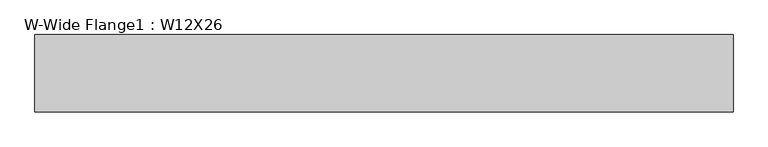
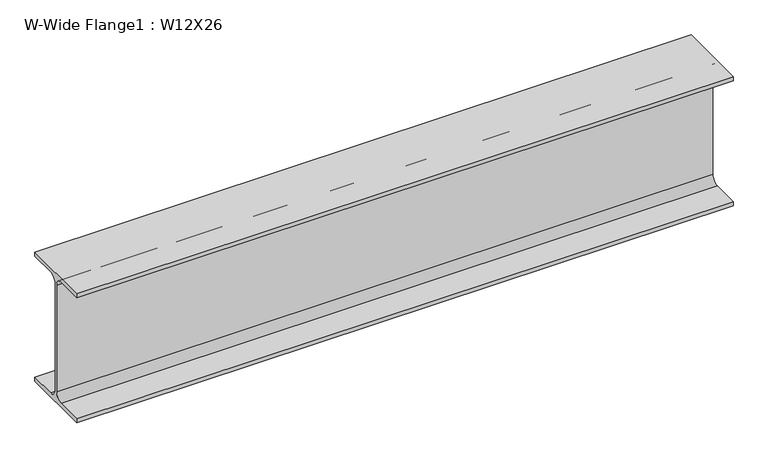
"""IFC4 building model written with IfcOpenShell, lengths in millimetres: beam geometry, W-Wide Flange1 : W12X26."""

from ifc_helpers import new_model, si_unit, point, frame, frame_2d, origin, place, context, project, spatial, polyline, circle_curve, trimmed, segment, composite_curve, outline, extrude, source, transform, mapped, element, save


def w_wide_flange1_w12x26_51e5bc3b(model_context):
    return source(origin(), model_context, "Body", "SweptSolid", [
        extrude(outline(composite_curve([segment(polyline([(82.423, -145.288), (82.423, -154.94), (-82.423, -154.94), (-82.423, -145.288), (-20.2565, -145.288)]), True, "CONTINUOUS"), segment(trimmed(circle_curve(frame_2d((-20.2565, -127.9525)), 17.3355), [point((-20.2565, -145.288))], [point((-2.921, -127.9525))], True, "CARTESIAN"), True, "CONTINUOUS"), segment(polyline([(-2.921, -127.9525), (-2.921, 127.9525)]), True, "CONTINUOUS"), segment(trimmed(circle_curve(frame_2d((-20.2565, 127.9525)), 17.3355), [point((-2.921, 127.9525))], [point((-20.2565, 145.288))], True, "CARTESIAN"), True, "CONTINUOUS"), segment(polyline([(-20.2565, 145.288), (-82.423, 145.288), (-82.423, 154.94), (82.423, 154.94), (82.423, 145.288), (20.2565, 145.288)]), True, "CONTINUOUS"), segment(trimmed(circle_curve(frame_2d((20.2565, 127.9525)), 17.3355), [point((20.2565, 145.288))], [point((2.921, 127.9525))], True, "CARTESIAN"), True, "CONTINUOUS"), segment(polyline([(2.921, 127.9525), (2.921, -127.9525)]), True, "CONTINUOUS"), segment(trimmed(circle_curve(frame_2d((20.2565, -127.9525)), 17.3355), [point((2.921, -127.9525))], [point((20.2565, -145.288))], True, "CARTESIAN"), True, "CONTINUOUS"), segment(polyline([(20.2565, -145.288), (82.423, -145.288)]), True, "CONTINUOUS")], self_intersect=False)), frame((-697.175026, 0.0, 0.0), z_axis=(1.0, 0.0, 0.0), x_axis=(0.0, 1.0, 0.0)), (0.0, 0.0, 1.0), 1490.8851174),
    ])


if __name__ == "__main__":
    model = new_model("IFC4")
    model_context = context("Model", 3, world=origin())
    ifc_project = project(units=[si_unit("LENGTHUNIT", "METRE", prefix="MILLI")], contexts=[model_context])
    site = spatial("IfcSite", under=ifc_project)
    building = spatial("IfcBuilding", under=site)
    placement = place(None, origin())
    w_wide_flange1_w12x26_shape = w_wide_flange1_w12x26_51e5bc3b(model_context)
    element("IfcBeam", 1, ObjectType="W-Wide Flange1 : W12X26", at=placement, inside=building, context=model_context, shape_type="MappedRepresentation", body=[
        mapped(w_wide_flange1_w12x26_shape, transform((0.0, 0.0, 0.0), x_axis=(1.0, 0.0, 0.0), y_axis=(0.0, 1.0, 0.0), z_axis=(0.0, 0.0, 1.0))),
    ])
    save(model, "model.ifc")

# Revit data of these elements
# Type "W-Wide Flange1 : W12X26"
#   Assembly Code = "B10"
#   W = 26
#   Start Extension Calculation [instance default] = 10' - 0"
#   Start Extension [instance default] = -0' - 0 1/2"
#   End Extension Calculation [instance default] = 10' - 0"
#   End Extension [instance default] = -0' - 0 1/2"
#   Length [instance default] = 5' - 0"
#   bf = 0' - 6.49"
#   d = 1' - 0.2"
#   k = 0' - 1 1/16"
#   k2 = 0' - 0.6825"
#   tf = 0' - 0.38"
#   tw = 0' - 0.23"
#   A = 0.053125 SF
#   Structural Material [instance default] = Metal - Steel - ASTM A992
# Element 1 (IfcBeam, "W-Wide Flange1 : W12X26")
#   Materials on its faces: "Metal - Steel - ASTM A992"
# Materials
#   "Metal - Steel - ASTM A992": class "Metal", colour RGB 199 199 199, transparency 0
